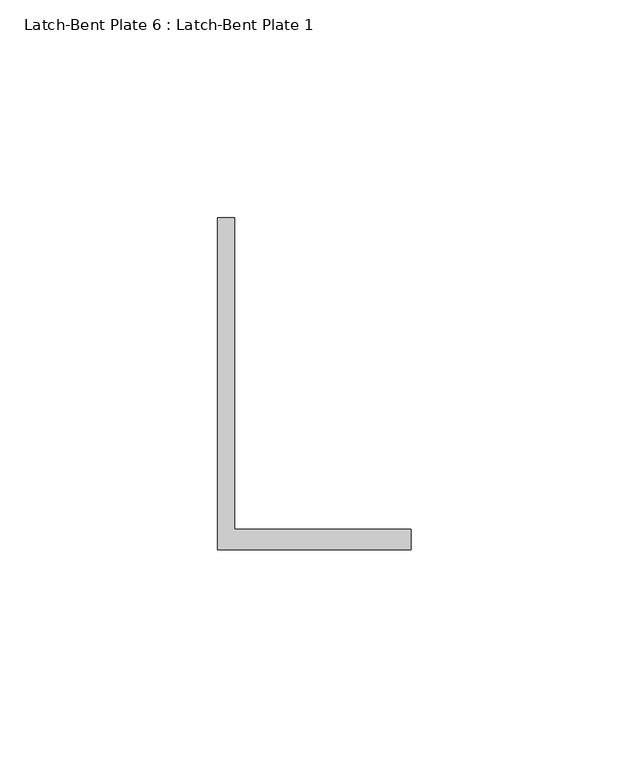
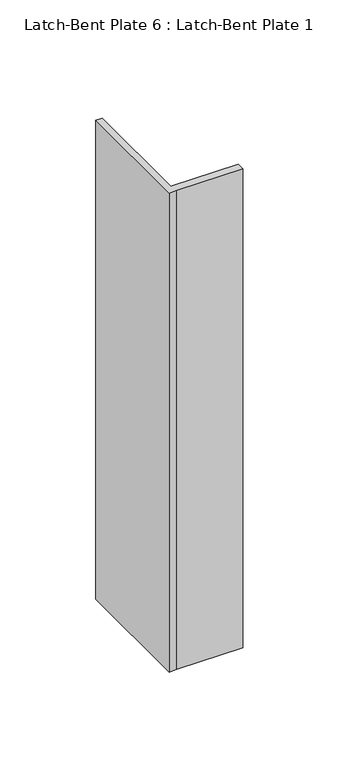
"""IFC4 building model written with IfcOpenShell, lengths in millimetres: proxy geometry, Latch-Bent Plate 6 : Latch-Bent Plate 1."""

from ifc_helpers import new_model, si_unit, frame, origin, place, context, project, spatial, polyline, outline, extrude, source, transform, mapped, element, save


def latch_bent_plate_6_latch_bent_plate_1_8bdba4d9(model_context):
    return source(origin(), model_context, "Body", "SweptSolid", [
        extrude(outline(polyline([(587327.0060739, -535201.5663841), (587322.2435739, -535201.5663841), (587322.2435739, -535125.3663841), (587326.1141748, -535125.3663841), (587326.1141748, -535196.8038841), (587366.6808739, -535196.8038841), (587366.6808739, -535201.5663841), (587327.0060739, -535201.5663841)])), frame((0.0, 0.0, 50.8), z_axis=(0.0, 0.0, 1.0), x_axis=(1.0, 0.0, 0.0)), (0.0, 0.0, 1.0), 304.8),
    ])


if __name__ == "__main__":
    model = new_model("IFC4")
    model_context = context("Model", 3, world=origin())
    ifc_project = project(units=[si_unit("LENGTHUNIT", "METRE", prefix="MILLI")], contexts=[model_context])
    site = spatial("IfcSite", under=ifc_project)
    building = spatial("IfcBuilding", under=site)
    placement = place(None, origin())
    latch_bent_plate_6_latch_bent_plate_1_shape = latch_bent_plate_6_latch_bent_plate_1_8bdba4d9(model_context)
    element("IfcBuildingElementProxy", 1, Name="Latch-Bent Plate 6 : Latch-Bent Plate 1", ObjectType="Latch-Bent Plate 6 : Latch-Bent Plate 1", at=placement, inside=building, context=model_context, shape_type="MappedRepresentation", body=[
        mapped(latch_bent_plate_6_latch_bent_plate_1_shape, transform((0.0, 0.0, 0.0), x_axis=(1.0, 0.0, 0.0), y_axis=(0.0, 1.0, 0.0), z_axis=(0.0, 0.0, 1.0))),
    ])
    save(model, "model.ifc")

# Revit data of these elements
# Element 1 (IfcBuildingElementProxy, "Latch-Bent Plate 6 : Latch-Bent Plate 1")
#   Materials on its faces: "GALV. GATE LATCH"
# Materials
#   "GALV. GATE LATCH": class "Metal", colour RGB 189 187 185, transparency 0, Description = "Carbon steel", Cost = 0
